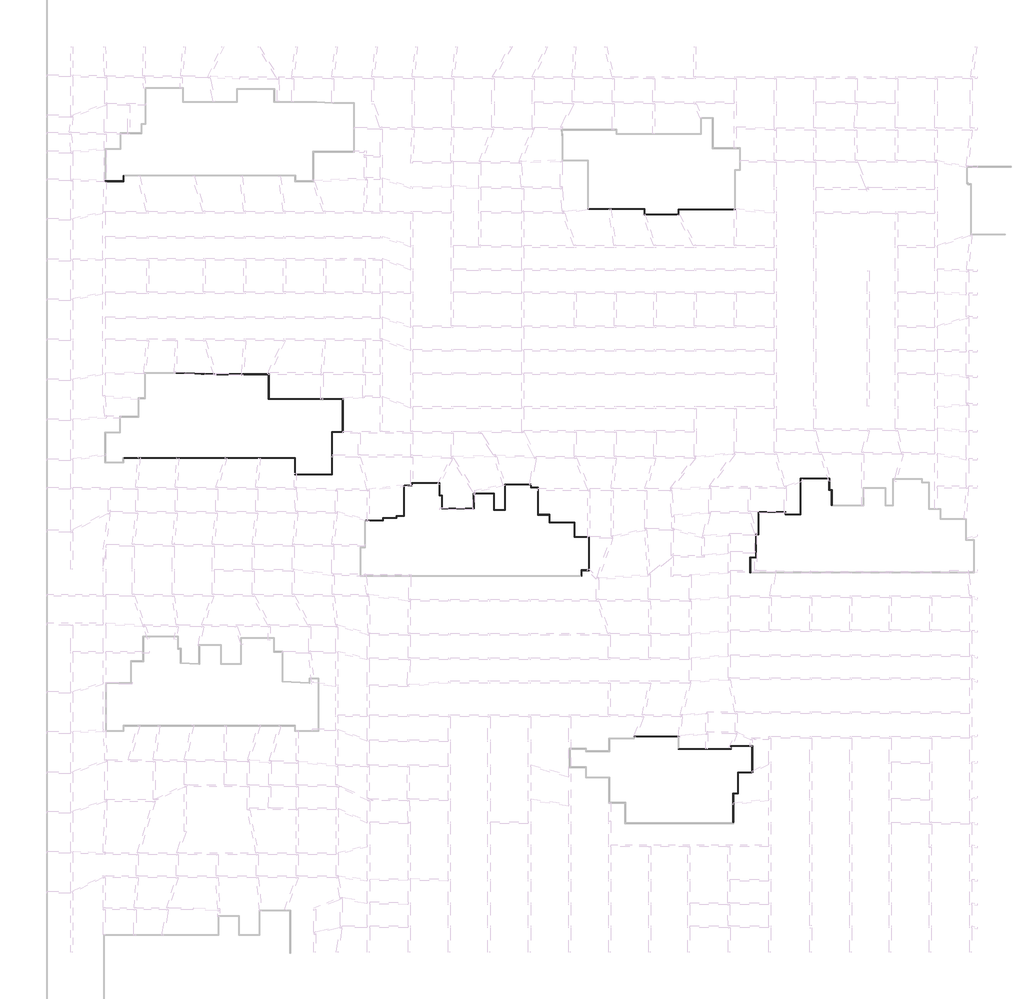
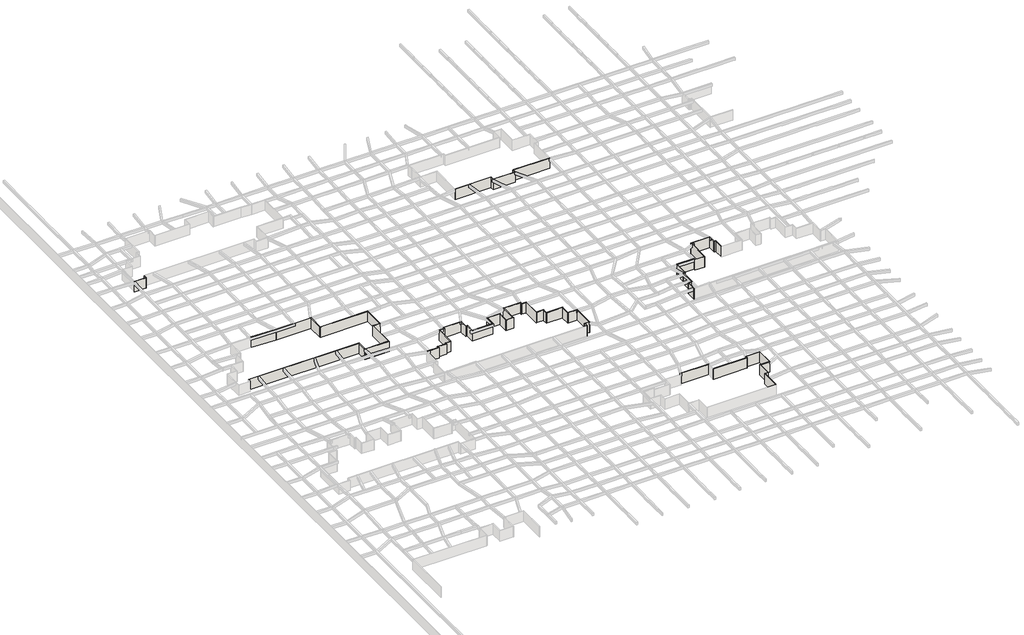
# One storey, part 6 of 45: 69 walls.
"""IFC4 building model written with IfcOpenShell, lengths in millimetres."""

from ifc_helpers import new_model, si_unit, origin, origin_with_axes, place, context, project, spatial, polyline, outline, extrude, faceted_brep, element, save

model = new_model("IFC4")

# Units and contexts
model_context = context("Model", 3, world=origin())
ifc_project = project(units=[si_unit("LENGTHUNIT", "METRE", prefix="MILLI")], contexts=[model_context])

# Site, building, storey
site = spatial("IfcSite", under=ifc_project)
building = spatial("IfcBuilding", under=site)
storey = spatial("IfcBuildingStorey", under=building, Name="户型图", Elevation=0.0)

# Walls
placement = place(None, origin())
element("IfcWall", 1, ObjectType="所有墙体", at=placement, inside=storey, context=model_context, shape_type="Brep", body=[
    faceted_brep([(-140203.5692432, 133175.8564831, 0.0), (-140203.5692432, 132195.8564831, 0.0), (-140203.5692432, 132075.8564831, 0.0), (-140203.5692432, 132075.8564831, 3300.0), (-140203.5692432, 132195.8564831, 3300.0), (-140203.5692432, 133175.8564831, 3300.0), (-140083.5692432, 133175.8564831, 0.0), (-140083.5692432, 133175.8564831, 3300.0), (-140083.5692432, 132075.8564831, 3300.0), (-140083.5692432, 132075.8564831, 0.0)], [[[0, 1, 2, 3, 4, 5]], [[6, 7, 8, 9]], [[2, 1, 0, 6, 9]], [[5, 4, 3, 8, 7]], [[0, 5, 7, 6]], [[3, 2, 9, 8]]]),
])
element("IfcWall", 2, ObjectType="所有墙体", at=placement, inside=storey, context=model_context, shape_type="Brep", body=[
    faceted_brep([(-140203.5692432, 132195.8564831, 0.0), (-143583.5692432, 132195.8564831, 0.0), (-143703.5692432, 132195.8564831, 0.0), (-143703.5692432, 132195.8564831, 3300.0), (-143583.5692432, 132195.8564831, 3300.0), (-140203.5692432, 132195.8564831, 3300.0), (-140203.5692432, 132075.8564831, 0.0), (-140203.5692432, 132075.8564831, 3300.0), (-143703.5692432, 132075.8564831, 3300.0), (-143703.5692432, 132075.8564831, 0.0)], [[[0, 1, 2, 3, 4, 5]], [[6, 7, 8, 9]], [[2, 1, 0, 6, 9]], [[5, 4, 3, 8, 7]], [[0, 5, 7, 6]], [[3, 2, 9, 8]]]),
])
element("IfcWall", 3, ObjectType="所有墙体", at=placement, inside=storey, context=model_context, shape_type="Brep", body=[
    faceted_brep([(-140131.3875586, 78294.2865852, 0.0), (-106851.3875586, 78294.2865852, 0.0), (-106731.3875586, 78294.2865852, 0.0), (-106731.3875586, 78294.2865852, 3300.0), (-106851.3875586, 78294.2865852, 3300.0), (-140131.3875586, 78294.2865852, 3300.0), (-140131.3875586, 78414.2865852, 0.0), (-140131.3875586, 78414.2865852, 3300.0), (-106731.3875586, 78414.2865852, 3300.0), (-106731.3875586, 78414.2865852, 0.0)], [[[0, 1, 2, 3, 4, 5]], [[6, 7, 8, 9]], [[2, 1, 0, 6, 9]], [[5, 4, 3, 8, 7]], [[0, 5, 7, 6]], [[3, 2, 9, 8]]]),
])
element("IfcWall", 4, ObjectType="所有墙体", at=placement, inside=storey, context=model_context, shape_type="Brep", body=[
    faceted_brep([(-106851.3875586, 78294.2865852, 0.0), (-106851.3875586, 75094.2865852, 0.0), (-106851.3875586, 75094.2865852, 3300.0), (-106851.3875586, 78294.2865852, 3300.0), (-106731.3875586, 78294.2865852, 0.0), (-106731.3875586, 78294.2865852, 3300.0), (-106731.3875586, 75214.2865852, 3300.0), (-106731.3875586, 75094.2865852, 3300.0), (-106731.3875586, 75094.2865852, 0.0), (-106731.3875586, 75214.2865852, 0.0)], [[[0, 1, 2, 3]], [[4, 5, 6, 7, 8, 9]], [[1, 0, 4, 9, 8]], [[3, 2, 7, 6, 5]], [[0, 3, 5, 4]], [[2, 1, 8, 7]]]),
])
element("IfcWall", 5, ObjectType="所有墙体", at=placement, inside=storey, context=model_context, shape_type="Brep", body=[
    faceted_brep([(-106731.3875586, 75094.2865852, 0.0), (-99531.3875586, 75094.2865852, 0.0), (-99531.3875586, 75094.2865852, 3300.0), (-106731.3875586, 75094.2865852, 3300.0), (-106731.3875586, 75214.2865852, 0.0), (-106731.3875586, 75214.2865852, 3300.0), (-99651.3875586, 75214.2865852, 3300.0), (-99531.3875586, 75214.2865852, 3300.0), (-99531.3875586, 75214.2865852, 0.0), (-99651.3875586, 75214.2865852, 0.0)], [[[0, 1, 2, 3]], [[4, 5, 6, 7, 8, 9]], [[1, 0, 4, 9, 8]], [[3, 2, 7, 6, 5]], [[0, 3, 5, 4]], [[2, 1, 8, 7]]]),
])
element("IfcWall", 6, ObjectType="所有墙体", at=placement, inside=storey, context=model_context, shape_type="Brep", body=[
    faceted_brep([(-99531.3875586, 75214.2865852, 0.0), (-99531.3875586, 83294.2865852, 0.0), (-99531.3875586, 83414.2865852, 0.0), (-99531.3875586, 83414.2865852, 3300.0), (-99531.3875586, 83294.2865852, 3300.0), (-99531.3875586, 75214.2865852, 3300.0), (-99651.3875586, 75214.2865852, 0.0), (-99651.3875586, 75214.2865852, 3300.0), (-99651.3875586, 83414.2865852, 3300.0), (-99651.3875586, 83414.2865852, 0.0)], [[[0, 1, 2, 3, 4, 5]], [[6, 7, 8, 9]], [[2, 1, 0, 6, 9]], [[5, 4, 3, 8, 7]], [[0, 5, 7, 6]], [[3, 2, 9, 8]]]),
])
element("IfcWall", 7, ObjectType="所有墙体", at=placement, inside=storey, context=model_context, shape_type="Brep", body=[
    faceted_brep([(-99531.3875586, 83294.2865852, 0.0), (-97431.3875586, 83294.2865852, 0.0), (-97431.3875586, 83294.2865852, 3300.0), (-99531.3875586, 83294.2865852, 3300.0), (-99531.3875586, 83414.2865852, 0.0), (-99531.3875586, 83414.2865852, 3300.0), (-97551.3875586, 83414.2865852, 3300.0), (-97431.3875586, 83414.2865852, 3300.0), (-97431.3875586, 83414.2865852, 0.0), (-97551.3875586, 83414.2865852, 0.0)], [[[0, 1, 2, 3]], [[4, 5, 6, 7, 8, 9]], [[1, 0, 4, 9, 8]], [[3, 2, 7, 6, 5]], [[0, 3, 5, 4]], [[2, 1, 8, 7]]]),
])
element("IfcWall", 8, ObjectType="所有墙体", at=placement, inside=storey, context=model_context, shape_type="Brep", body=[
    faceted_brep([(-97431.3875586, 83414.2865852, 0.0), (-97431.3875586, 89872.92078, 0.0), (-97431.3875586, 89872.92078, 3300.0), (-97431.3875586, 83414.2865852, 3300.0), (-97551.3875586, 83414.2865852, 0.0), (-97551.3875586, 83414.2865852, 3300.0), (-97551.3875586, 89752.92078, 3300.0), (-97551.3875586, 89872.92078, 3300.0), (-97551.3875586, 89872.92078, 0.0), (-97551.3875586, 89752.92078, 0.0)], [[[0, 1, 2, 3]], [[4, 5, 6, 7, 8, 9]], [[1, 0, 4, 9, 8]], [[3, 2, 7, 6, 5]], [[0, 3, 5, 4]], [[2, 1, 8, 7]]]),
])
element("IfcWall", 9, ObjectType="所有墙体", at=placement, inside=storey, context=model_context, shape_type="Brep", body=[
    faceted_brep([(-97551.3875586, 89872.92078, 0.0), (-111831.3875586, 89872.92078, 0.0), (-111951.3875586, 89872.92078, 0.0), (-111951.3875586, 89872.92078, 3300.0), (-111831.3875586, 89872.92078, 3300.0), (-97551.3875586, 89872.92078, 3300.0), (-97551.3875586, 89752.92078, 0.0), (-97551.3875586, 89752.92078, 3300.0), (-111951.3875586, 89752.92078, 3300.0), (-111951.3875586, 89752.92078, 0.0)], [[[0, 1, 2, 3, 4, 5]], [[6, 7, 8, 9]], [[2, 1, 0, 6, 9]], [[5, 4, 3, 8, 7]], [[0, 5, 7, 6]], [[3, 2, 9, 8]]]),
])
element("IfcWall", 10, ObjectType="所有墙体", at=placement, inside=storey, context=model_context, shape_type="Brep", body=[
    faceted_brep([(-111831.3875586, 89872.92078, 0.0), (-111831.3875586, 94672.92078, 0.0), (-111831.3875586, 94672.92078, 3300.0), (-111831.3875586, 89872.92078, 3300.0), (-111951.3875586, 89872.92078, 0.0), (-111951.3875586, 89872.92078, 3300.0), (-111951.3875586, 94552.92078, 3300.0), (-111951.3875586, 94672.92078, 3300.0), (-111951.3875586, 94672.92078, 0.0), (-111951.3875586, 94552.92078, 0.0)], [[[0, 1, 2, 3]], [[4, 5, 6, 7, 8, 9]], [[1, 0, 4, 9, 8]], [[3, 2, 7, 6, 5]], [[0, 3, 5, 4]], [[2, 1, 8, 7]]]),
])
element("IfcWall", 11, ObjectType="所有墙体", at=placement, inside=storey, context=model_context, shape_type="SweptSolid", body=[
    extrude(outline(polyline([(-122490.3402547, 94672.92078), (-111951.3875586, 94672.92078), (-111951.3875586, 94552.92078), (-122492.4348625, 94552.92078), (-122490.3402547, 94672.92078)])), origin_with_axes(), (0.0, 0.0, 1.0), 3300.0),
])
element("IfcWall", 12, ObjectType="所有墙体", at=placement, inside=storey, context=model_context, shape_type="SweptSolid", body=[
    extrude(outline(polyline([(-129985.7714573, 94934.6670053), (-122490.3402547, 94672.92078), (-122492.4348625, 94552.92078), (-129987.8660651, 94814.6670053), (-129985.7714573, 94934.6670053)])), origin_with_axes(), (0.0, 0.0, 1.0), 3300.0),
])
element("IfcWall", 13, ObjectType="所有墙体", at=placement, inside=storey, context=model_context, shape_type="Brep", body=[
    faceted_brep([(-49787.1090692, 126702.9605472, 0.0), (-38907.1090692, 126702.9605472, 0.0), (-38787.1090692, 126702.9605472, 0.0), (-38787.1090692, 126702.9605472, 3300.0), (-38907.1090692, 126702.9605472, 3300.0), (-49787.1090692, 126702.9605472, 3300.0), (-49787.1090692, 126822.9605472, 0.0), (-49787.1090692, 126822.9605472, 3300.0), (-38787.1090692, 126822.9605472, 3300.0), (-38787.1090692, 126822.9605472, 0.0)], [[[0, 1, 2, 3, 4, 5]], [[6, 7, 8, 9]], [[2, 1, 0, 6, 9]], [[5, 4, 3, 8, 7]], [[0, 5, 7, 6]], [[3, 2, 9, 8]]]),
])
element("IfcWall", 14, ObjectType="所有墙体", at=placement, inside=storey, context=model_context, shape_type="Brep", body=[
    faceted_brep([(-38907.1090692, 126702.9605472, 0.0), (-38907.1090692, 125602.9605472, 0.0), (-38907.1090692, 125602.9605472, 3300.0), (-38907.1090692, 126702.9605472, 3300.0), (-38787.1090692, 126702.9605472, 0.0), (-38787.1090692, 126702.9605472, 3300.0), (-38787.1090692, 125722.9605472, 3300.0), (-38787.1090692, 125602.9605472, 3300.0), (-38787.1090692, 125602.9605472, 0.0), (-38787.1090692, 125722.9605472, 0.0)], [[[0, 1, 2, 3]], [[4, 5, 6, 7, 8, 9]], [[1, 0, 4, 9, 8]], [[3, 2, 7, 6, 5]], [[0, 3, 5, 4]], [[2, 1, 8, 7]]]),
])
element("IfcWall", 15, ObjectType="所有墙体", at=placement, inside=storey, context=model_context, shape_type="Brep", body=[
    faceted_brep([(-38787.1090692, 125602.9605472, 0.0), (-32187.1090692, 125602.9605472, 0.0), (-32187.1090692, 125602.9605472, 3300.0), (-38787.1090692, 125602.9605472, 3300.0), (-38787.1090692, 125722.9605472, 0.0), (-38787.1090692, 125722.9605472, 3300.0), (-32307.1090692, 125722.9605472, 3300.0), (-32187.1090692, 125722.9605472, 3300.0), (-32187.1090692, 125722.9605472, 0.0), (-32307.1090692, 125722.9605472, 0.0)], [[[0, 1, 2, 3]], [[4, 5, 6, 7, 8, 9]], [[1, 0, 4, 9, 8]], [[3, 2, 7, 6, 5]], [[0, 3, 5, 4]], [[2, 1, 8, 7]]]),
])
element("IfcWall", 16, ObjectType="所有墙体", at=placement, inside=storey, context=model_context, shape_type="Brep", body=[
    faceted_brep([(-32187.1090692, 125722.9605472, 0.0), (-32187.1090692, 126602.9605472, 0.0), (-32187.1090692, 126722.9605472, 0.0), (-32187.1090692, 126722.9605472, 3300.0), (-32187.1090692, 126602.9605472, 3300.0), (-32187.1090692, 125722.9605472, 3300.0), (-32307.1090692, 125722.9605472, 0.0), (-32307.1090692, 125722.9605472, 3300.0), (-32307.1090692, 126722.9605472, 3300.0), (-32307.1090692, 126722.9605472, 0.0)], [[[0, 1, 2, 3, 4, 5]], [[6, 7, 8, 9]], [[2, 1, 0, 6, 9]], [[5, 4, 3, 8, 7]], [[0, 5, 7, 6]], [[3, 2, 9, 8]]]),
])
element("IfcWall", 17, ObjectType="所有墙体", at=placement, inside=storey, context=model_context, shape_type="Brep", body=[
    faceted_brep([(-32187.1090692, 126602.9605472, 0.0), (-21187.1090692, 126602.9605472, 0.0), (-21187.1090692, 126602.9605472, 3300.0), (-32187.1090692, 126602.9605472, 3300.0), (-32187.1090692, 126722.9605472, 0.0), (-32187.1090692, 126722.9605472, 3300.0), (-21307.1090692, 126722.9605472, 3300.0), (-21187.1090692, 126722.9605472, 3300.0), (-21187.1090692, 126722.9605472, 0.0), (-21307.1090692, 126722.9605472, 0.0)], [[[0, 1, 2, 3]], [[4, 5, 6, 7, 8, 9]], [[1, 0, 4, 9, 8]], [[3, 2, 7, 6, 5]], [[0, 3, 5, 4]], [[2, 1, 8, 7]]]),
])
element("IfcWall", 18, ObjectType="所有墙体", at=placement, inside=storey, context=model_context, shape_type="Brep", body=[
    faceted_brep([(-93093.897353, 66089.1206587, 0.0), (-89610.9508463, 66089.1206587, 0.0), (-89610.9508463, 66089.1206587, 3300.0), (-93093.897353, 66089.1206587, 3300.0), (-93093.897353, 66209.1206587, 0.0), (-93093.897353, 66209.1206587, 3300.0), (-89730.9508463, 66209.1206587, 3300.0), (-89610.9508463, 66209.1206587, 3300.0), (-89610.9508463, 66209.1206587, 0.0), (-89730.9508463, 66209.1206587, 0.0)], [[[0, 1, 2, 3]], [[4, 5, 6, 7, 8, 9]], [[1, 0, 4, 9, 8]], [[3, 2, 7, 6, 5]], [[2, 1, 8, 7]], [[0, 3, 5, 4]]]),
])
element("IfcWall", 19, ObjectType="所有墙体", at=placement, inside=storey, context=model_context, shape_type="Brep", body=[
    faceted_brep([(-89610.9508463, 66209.1206587, 0.0), (-89610.9508463, 66589.1206587, 0.0), (-89610.9508463, 66709.1206587, 0.0), (-89610.9508463, 66709.1206587, 3300.0), (-89610.9508463, 66589.1206587, 3300.0), (-89610.9508463, 66209.1206587, 3300.0), (-89730.9508463, 66209.1206587, 0.0), (-89730.9508463, 66209.1206587, 3300.0), (-89730.9508463, 66709.1206587, 3300.0), (-89730.9508463, 66709.1206587, 0.0)], [[[0, 1, 2, 3, 4, 5]], [[6, 7, 8, 9]], [[2, 1, 0, 6, 9]], [[5, 4, 3, 8, 7]], [[0, 5, 7, 6]], [[3, 2, 9, 8]]]),
])
element("IfcWall", 20, ObjectType="所有墙体", at=placement, inside=storey, context=model_context, shape_type="Brep", body=[
    faceted_brep([(-89610.9508463, 66589.1206587, 0.0), (-87010.9508463, 66589.1206587, 0.0), (-87010.9508463, 66589.1206587, 3300.0), (-89610.9508463, 66589.1206587, 3300.0), (-89610.9508463, 66709.1206587, 0.0), (-89610.9508463, 66709.1206587, 3300.0), (-87130.9508463, 66709.1206587, 3300.0), (-87010.9508463, 66709.1206587, 3300.0), (-87010.9508463, 66709.1206587, 0.0), (-87130.9508463, 66709.1206587, 0.0)], [[[0, 1, 2, 3]], [[4, 5, 6, 7, 8, 9]], [[1, 0, 4, 9, 8]], [[3, 2, 7, 6, 5]], [[0, 3, 5, 4]], [[2, 1, 8, 7]]]),
])
element("IfcWall", 21, ObjectType="所有墙体", at=placement, inside=storey, context=model_context, shape_type="Brep", body=[
    faceted_brep([(-87010.9508463, 66709.1206587, 0.0), (-87010.9508463, 66989.1206587, 0.0), (-87010.9508463, 67109.1206587, 0.0), (-87010.9508463, 67109.1206587, 3300.0), (-87010.9508463, 66989.1206587, 3300.0), (-87010.9508463, 66709.1206587, 3300.0), (-87130.9508463, 66709.1206587, 0.0), (-87130.9508463, 66709.1206587, 3300.0), (-87130.9508463, 67109.1206587, 3300.0), (-87130.9508463, 67109.1206587, 0.0)], [[[0, 1, 2, 3, 4, 5]], [[6, 7, 8, 9]], [[2, 1, 0, 6, 9]], [[5, 4, 3, 8, 7]], [[0, 5, 7, 6]], [[3, 2, 9, 8]]]),
])
element("IfcWall", 22, ObjectType="所有墙体", at=placement, inside=storey, context=model_context, shape_type="Brep", body=[
    faceted_brep([(-87010.9508463, 66989.1206587, 0.0), (-85510.9508463, 66989.1206587, 0.0), (-85510.9508463, 66989.1206587, 3300.0), (-87010.9508463, 66989.1206587, 3300.0), (-87010.9508463, 67109.1206587, 0.0), (-87010.9508463, 67109.1206587, 3300.0), (-85630.9508463, 67109.1206587, 3300.0), (-85510.9508463, 67109.1206587, 3300.0), (-85510.9508463, 67109.1206587, 0.0), (-85630.9508463, 67109.1206587, 0.0)], [[[0, 1, 2, 3]], [[4, 5, 6, 7, 8, 9]], [[1, 0, 4, 9, 8]], [[3, 2, 7, 6, 5]], [[0, 3, 5, 4]], [[2, 1, 8, 7]]]),
])
element("IfcWall", 23, ObjectType="所有墙体", at=placement, inside=storey, context=model_context, shape_type="Brep", body=[
    faceted_brep([(-85510.9508463, 67109.1206587, 0.0), (-85510.9508463, 72887.1913736, 0.0), (-85510.9508463, 73007.1913736, 0.0), (-85510.9508463, 73007.1913736, 3300.0), (-85510.9508463, 72887.1913736, 3300.0), (-85510.9508463, 67109.1206587, 3300.0), (-85630.9508463, 67109.1206587, 0.0), (-85630.9508463, 67109.1206587, 3300.0), (-85630.9508463, 73007.1913736, 3300.0), (-85630.9508463, 73007.1913736, 0.0)], [[[0, 1, 2, 3, 4, 5]], [[6, 7, 8, 9]], [[2, 1, 0, 6, 9]], [[5, 4, 3, 8, 7]], [[0, 5, 7, 6]], [[3, 2, 9, 8]]]),
])
element("IfcWall", 24, ObjectType="所有墙体", at=placement, inside=storey, context=model_context, shape_type="Brep", body=[
    faceted_brep([(-85510.9508463, 72887.1913736, 0.0), (-84010.9508463, 72887.1913736, 0.0), (-84010.9508463, 72887.1913736, 3300.0), (-85510.9508463, 72887.1913736, 3300.0), (-85510.9508463, 73007.1913736, 0.0), (-85510.9508463, 73007.1913736, 3300.0), (-84130.9508463, 73007.1913736, 3300.0), (-84010.9508463, 73007.1913736, 3300.0), (-84010.9508463, 73007.1913736, 0.0), (-84130.9508463, 73007.1913736, 0.0)], [[[0, 1, 2, 3]], [[4, 5, 6, 7, 8, 9]], [[1, 0, 4, 9, 8]], [[3, 2, 7, 6, 5]], [[0, 3, 5, 4]], [[2, 1, 8, 7]]]),
])
element("IfcWall", 25, ObjectType="所有墙体", at=placement, inside=storey, context=model_context, shape_type="Brep", body=[
    faceted_brep([(-84010.9508463, 73007.1913736, 0.0), (-84010.9508463, 73387.1913736, 0.0), (-84010.9508463, 73507.1913736, 0.0), (-84010.9508463, 73507.1913736, 3300.0), (-84010.9508463, 73387.1913736, 3300.0), (-84010.9508463, 73007.1913736, 3300.0), (-84130.9508463, 73007.1913736, 0.0), (-84130.9508463, 73007.1913736, 3300.0), (-84130.9508463, 73507.1913736, 3300.0), (-84130.9508463, 73507.1913736, 0.0)], [[[0, 1, 2, 3, 4, 5]], [[6, 7, 8, 9]], [[2, 1, 0, 6, 9]], [[5, 4, 3, 8, 7]], [[0, 5, 7, 6]], [[3, 2, 9, 8]]]),
])
element("IfcWall", 26, ObjectType="所有墙体", at=placement, inside=storey, context=model_context, shape_type="Brep", body=[
    faceted_brep([(-84010.9508463, 73387.1913736, 0.0), (-78767.8659344, 73387.1913736, 0.0), (-78647.8659344, 73387.1913736, 0.0), (-78647.8659344, 73387.1913736, 3300.0), (-78767.8659344, 73387.1913736, 3300.0), (-84010.9508463, 73387.1913736, 3300.0), (-84010.9508463, 73507.1913736, 0.0), (-84010.9508463, 73507.1913736, 3300.0), (-78647.8659344, 73507.1913736, 3300.0), (-78647.8659344, 73507.1913736, 0.0)], [[[0, 1, 2, 3, 4, 5]], [[6, 7, 8, 9]], [[2, 1, 0, 6, 9]], [[5, 4, 3, 8, 7]], [[0, 5, 7, 6]], [[3, 2, 9, 8]]]),
])
element("IfcWall", 27, ObjectType="所有墙体", at=placement, inside=storey, context=model_context, shape_type="Brep", body=[
    faceted_brep([(-78767.8659344, 73387.1913736, 0.0), (-78767.8659344, 70987.1913736, 0.0), (-78767.8659344, 70987.1913736, 3300.0), (-78767.8659344, 73387.1913736, 3300.0), (-78647.8659344, 73387.1913736, 0.0), (-78647.8659344, 73387.1913736, 3300.0), (-78647.8659344, 71107.1913736, 3300.0), (-78647.8659344, 70987.1913736, 3300.0), (-78647.8659344, 70987.1913736, 0.0), (-78647.8659344, 71107.1913736, 0.0)], [[[0, 1, 2, 3]], [[4, 5, 6, 7, 8, 9]], [[1, 0, 4, 9, 8]], [[3, 2, 7, 6, 5]], [[0, 3, 5, 4]], [[2, 1, 8, 7]]]),
])
element("IfcWall", 28, ObjectType="所有墙体", at=placement, inside=storey, context=model_context, shape_type="Brep", body=[
    faceted_brep([(-78647.8659344, 70987.1913736, 0.0), (-78267.8659344, 70987.1913736, 0.0), (-78147.8659344, 70987.1913736, 0.0), (-78147.8659344, 70987.1913736, 3300.0), (-78267.8659344, 70987.1913736, 3300.0), (-78647.8659344, 70987.1913736, 3300.0), (-78647.8659344, 71107.1913736, 0.0), (-78647.8659344, 71107.1913736, 3300.0), (-78147.8659344, 71107.1913736, 3300.0), (-78147.8659344, 71107.1913736, 0.0)], [[[0, 1, 2, 3, 4, 5]], [[6, 7, 8, 9]], [[2, 1, 0, 6, 9]], [[5, 4, 3, 8, 7]], [[0, 5, 7, 6]], [[3, 2, 9, 8]]]),
])
element("IfcWall", 29, ObjectType="所有墙体", at=placement, inside=storey, context=model_context, shape_type="Brep", body=[
    faceted_brep([(-78267.8659344, 70987.1913736, 0.0), (-78267.8659344, 68427.6131193, 0.0), (-78267.8659344, 68427.6131193, 3300.0), (-78267.8659344, 70987.1913736, 3300.0), (-78147.8659344, 70987.1913736, 0.0), (-78147.8659344, 70987.1913736, 3300.0), (-78147.8659344, 68547.6131193, 3300.0), (-78147.8659344, 68427.6131193, 3300.0), (-78147.8659344, 68427.6131193, 0.0), (-78147.8659344, 68547.6131193, 0.0)], [[[0, 1, 2, 3]], [[4, 5, 6, 7, 8, 9]], [[1, 0, 4, 9, 8]], [[3, 2, 7, 6, 5]], [[0, 3, 5, 4]], [[2, 1, 8, 7]]]),
])
element("IfcWall", 30, ObjectType="所有墙体", at=placement, inside=storey, context=model_context, shape_type="Brep", body=[
    faceted_brep([(-78147.8659344, 68427.6131193, 0.0), (-71958.8192159, 68427.6131193, 0.0), (-71958.8192159, 68427.6131193, 3300.0), (-78147.8659344, 68427.6131193, 3300.0), (-78147.8659344, 68547.6131193, 0.0), (-78147.8659344, 68547.6131193, 3300.0), (-72078.8192159, 68547.6131193, 3300.0), (-71958.8192159, 68547.6131193, 3300.0), (-71958.8192159, 68547.6131193, 0.0), (-72078.8192159, 68547.6131193, 0.0)], [[[0, 1, 2, 3]], [[4, 5, 6, 7, 8, 9]], [[1, 0, 4, 9, 8]], [[3, 2, 7, 6, 5]], [[0, 3, 5, 4]], [[2, 1, 8, 7]]]),
])
element("IfcWall", 31, ObjectType="所有墙体", at=placement, inside=storey, context=model_context, shape_type="Brep", body=[
    faceted_brep([(-71958.8192159, 68547.6131193, 0.0), (-71958.8192159, 71355.8858644, 0.0), (-71958.8192159, 71475.8858644, 0.0), (-71958.8192159, 71475.8858644, 3300.0), (-71958.8192159, 71355.8858644, 3300.0), (-71958.8192159, 68547.6131193, 3300.0), (-72078.8192159, 68547.6131193, 0.0), (-72078.8192159, 68547.6131193, 3300.0), (-72078.8192159, 71475.8858644, 3300.0), (-72078.8192159, 71475.8858644, 0.0)], [[[0, 1, 2, 3, 4, 5]], [[6, 7, 8, 9]], [[2, 1, 0, 6, 9]], [[5, 4, 3, 8, 7]], [[0, 5, 7, 6]], [[3, 2, 9, 8]]]),
])
element("IfcWall", 32, ObjectType="所有墙体", at=placement, inside=storey, context=model_context, shape_type="Brep", body=[
    faceted_brep([(-71958.8192159, 71355.8858644, 0.0), (-68178.8192159, 71355.8858644, 0.0), (-68058.8192159, 71355.8858644, 0.0), (-68058.8192159, 71355.8858644, 3300.0), (-68178.8192159, 71355.8858644, 3300.0), (-71958.8192159, 71355.8858644, 3300.0), (-71958.8192159, 71475.8858644, 0.0), (-71958.8192159, 71475.8858644, 3300.0), (-68058.8192159, 71475.8858644, 3300.0), (-68058.8192159, 71475.8858644, 0.0)], [[[0, 1, 2, 3, 4, 5]], [[6, 7, 8, 9]], [[2, 1, 0, 6, 9]], [[5, 4, 3, 8, 7]], [[0, 5, 7, 6]], [[3, 2, 9, 8]]]),
])
element("IfcWall", 33, ObjectType="所有墙体", at=placement, inside=storey, context=model_context, shape_type="Brep", body=[
    faceted_brep([(-68178.8192159, 71355.8858644, 0.0), (-68178.8192159, 68155.8858644, 0.0), (-68178.8192159, 68155.8858644, 3300.0), (-68178.8192159, 71355.8858644, 3300.0), (-68058.8192159, 71355.8858644, 0.0), (-68058.8192159, 71355.8858644, 3300.0), (-68058.8192159, 68275.8858644, 3300.0), (-68058.8192159, 68155.8858644, 3300.0), (-68058.8192159, 68155.8858644, 0.0), (-68058.8192159, 68275.8858644, 0.0)], [[[0, 1, 2, 3]], [[4, 5, 6, 7, 8, 9]], [[1, 0, 4, 9, 8]], [[3, 2, 7, 6, 5]], [[0, 3, 5, 4]], [[2, 1, 8, 7]]]),
])
element("IfcWall", 34, ObjectType="所有墙体", at=placement, inside=storey, context=model_context, shape_type="Brep", body=[
    faceted_brep([(-68058.8192159, 68155.8858644, 0.0), (-65858.8192159, 68155.8858644, 0.0), (-65858.8192159, 68155.8858644, 3300.0), (-68058.8192159, 68155.8858644, 3300.0), (-68058.8192159, 68275.8858644, 0.0), (-68058.8192159, 68275.8858644, 3300.0), (-65978.8192159, 68275.8858644, 3300.0), (-65858.8192159, 68275.8858644, 3300.0), (-65858.8192159, 68275.8858644, 0.0), (-65978.8192159, 68275.8858644, 0.0)], [[[0, 1, 2, 3]], [[4, 5, 6, 7, 8, 9]], [[1, 0, 4, 9, 8]], [[3, 2, 7, 6, 5]], [[0, 3, 5, 4]], [[2, 1, 8, 7]]]),
])
element("IfcWall", 35, ObjectType="所有墙体", at=placement, inside=storey, context=model_context, shape_type="Brep", body=[
    faceted_brep([(-65858.8192159, 68275.8858644, 0.0), (-65858.8192159, 73135.9090851, 0.0), (-65858.8192159, 73255.9090851, 0.0), (-65858.8192159, 73255.9090851, 3300.0), (-65858.8192159, 73135.9090851, 3300.0), (-65858.8192159, 68275.8858644, 3300.0), (-65978.8192159, 68275.8858644, 0.0), (-65978.8192159, 68275.8858644, 3300.0), (-65978.8192159, 73255.9090851, 3300.0), (-65978.8192159, 73255.9090851, 0.0)], [[[0, 1, 2, 3, 4, 5]], [[6, 7, 8, 9]], [[2, 1, 0, 6, 9]], [[5, 4, 3, 8, 7]], [[0, 5, 7, 6]], [[3, 2, 9, 8]]]),
])
element("IfcWall", 36, ObjectType="所有墙体", at=placement, inside=storey, context=model_context, shape_type="Brep", body=[
    faceted_brep([(-65858.8192159, 73135.9090851, 0.0), (-60973.897353, 73135.9090851, 0.0), (-60853.897353, 73135.9090851, 0.0), (-60853.897353, 73135.9090851, 3300.0), (-60973.897353, 73135.9090851, 3300.0), (-65858.8192159, 73135.9090851, 3300.0), (-65858.8192159, 73255.9090851, 0.0), (-65858.8192159, 73255.9090851, 3300.0), (-60853.897353, 73255.9090851, 3300.0), (-60853.897353, 73255.9090851, 0.0)], [[[0, 1, 2, 3, 4, 5]], [[6, 7, 8, 9]], [[2, 1, 0, 6, 9]], [[5, 4, 3, 8, 7]], [[0, 5, 7, 6]], [[3, 2, 9, 8]]]),
])
element("IfcWall", 37, ObjectType="所有墙体", at=placement, inside=storey, context=model_context, shape_type="Brep", body=[
    faceted_brep([(-60973.897353, 73135.9090851, 0.0), (-60973.897353, 72535.9090851, 0.0), (-60973.897353, 72535.9090851, 3300.0), (-60973.897353, 73135.9090851, 3300.0), (-60853.897353, 73135.9090851, 0.0), (-60853.897353, 73135.9090851, 3300.0), (-60853.897353, 72655.9090851, 3300.0), (-60853.897353, 72535.9090851, 3300.0), (-60853.897353, 72535.9090851, 0.0), (-60853.897353, 72655.9090851, 0.0)], [[[0, 1, 2, 3]], [[4, 5, 6, 7, 8, 9]], [[1, 0, 4, 9, 8]], [[3, 2, 7, 6, 5]], [[0, 3, 5, 4]], [[2, 1, 8, 7]]]),
])
element("IfcWall", 38, ObjectType="所有墙体", at=placement, inside=storey, context=model_context, shape_type="Brep", body=[
    faceted_brep([(-60853.897353, 72535.9090851, 0.0), (-59573.897353, 72535.9090851, 0.0), (-59453.897353, 72535.9090851, 0.0), (-59453.897353, 72535.9090851, 3300.0), (-59573.897353, 72535.9090851, 3300.0), (-60853.897353, 72535.9090851, 3300.0), (-60853.897353, 72655.9090851, 0.0), (-60853.897353, 72655.9090851, 3300.0), (-59453.897353, 72655.9090851, 3300.0), (-59453.897353, 72655.9090851, 0.0)], [[[0, 1, 2, 3, 4, 5]], [[6, 7, 8, 9]], [[2, 1, 0, 6, 9]], [[5, 4, 3, 8, 7]], [[0, 5, 7, 6]], [[3, 2, 9, 8]]]),
])
element("IfcWall", 39, ObjectType="所有墙体", at=placement, inside=storey, context=model_context, shape_type="Brep", body=[
    faceted_brep([(-59573.897353, 72535.9090851, 0.0), (-59573.897353, 67235.9090851, 0.0), (-59573.897353, 67235.9090851, 3300.0), (-59573.897353, 72535.9090851, 3300.0), (-59453.897353, 72535.9090851, 0.0), (-59453.897353, 72535.9090851, 3300.0), (-59453.897353, 67355.9090851, 3300.0), (-59453.897353, 67235.9090851, 3300.0), (-59453.897353, 67235.9090851, 0.0), (-59453.897353, 67355.9090851, 0.0)], [[[0, 1, 2, 3]], [[4, 5, 6, 7, 8, 9]], [[1, 0, 4, 9, 8]], [[3, 2, 7, 6, 5]], [[0, 3, 5, 4]], [[2, 1, 8, 7]]]),
])
element("IfcWall", 40, ObjectType="所有墙体", at=placement, inside=storey, context=model_context, shape_type="Brep", body=[
    faceted_brep([(-59453.897353, 67235.9090851, 0.0), (-57373.897353, 67235.9090851, 0.0), (-57253.897353, 67235.9090851, 0.0), (-57253.897353, 67235.9090851, 3300.0), (-57373.897353, 67235.9090851, 3300.0), (-59453.897353, 67235.9090851, 3300.0), (-59453.897353, 67355.9090851, 0.0), (-59453.897353, 67355.9090851, 3300.0), (-57253.897353, 67355.9090851, 3300.0), (-57253.897353, 67355.9090851, 0.0)], [[[0, 1, 2, 3, 4, 5]], [[6, 7, 8, 9]], [[2, 1, 0, 6, 9]], [[5, 4, 3, 8, 7]], [[0, 5, 7, 6]], [[3, 2, 9, 8]]]),
])
element("IfcWall", 41, ObjectType="所有墙体", at=placement, inside=storey, context=model_context, shape_type="Brep", body=[
    faceted_brep([(-57373.897353, 67235.9090851, 0.0), (-57373.897353, 65735.9090851, 0.0), (-57373.897353, 65735.9090851, 3300.0), (-57373.897353, 67235.9090851, 3300.0), (-57253.897353, 67235.9090851, 0.0), (-57253.897353, 67235.9090851, 3300.0), (-57253.897353, 65855.9090851, 3300.0), (-57253.897353, 65735.9090851, 3300.0), (-57253.897353, 65735.9090851, 0.0), (-57253.897353, 65855.9090851, 0.0)], [[[0, 1, 2, 3]], [[4, 5, 6, 7, 8, 9]], [[1, 0, 4, 9, 8]], [[3, 2, 7, 6, 5]], [[0, 3, 5, 4]], [[2, 1, 8, 7]]]),
])
element("IfcWall", 42, ObjectType="所有墙体", at=placement, inside=storey, context=model_context, shape_type="Brep", body=[
    faceted_brep([(-57253.897353, 65735.9090851, 0.0), (-52473.897353, 65735.9090851, 0.0), (-52353.897353, 65735.9090851, 0.0), (-52353.897353, 65735.9090851, 3300.0), (-52473.897353, 65735.9090851, 3300.0), (-57253.897353, 65735.9090851, 3300.0), (-57253.897353, 65855.9090851, 0.0), (-57253.897353, 65855.9090851, 3300.0), (-52353.897353, 65855.9090851, 3300.0), (-52353.897353, 65855.9090851, 0.0)], [[[0, 1, 2, 3, 4, 5]], [[6, 7, 8, 9]], [[2, 1, 0, 6, 9]], [[5, 4, 3, 8, 7]], [[0, 5, 7, 6]], [[3, 2, 9, 8]]]),
])
element("IfcWall", 43, ObjectType="所有墙体", at=placement, inside=storey, context=model_context, shape_type="Brep", body=[
    faceted_brep([(-52473.897353, 65735.9090851, 0.0), (-52473.897353, 62935.9090851, 0.0), (-52473.897353, 62935.9090851, 3300.0), (-52473.897353, 65735.9090851, 3300.0), (-52353.897353, 65735.9090851, 0.0), (-52353.897353, 65735.9090851, 3300.0), (-52353.897353, 63055.9090851, 3300.0), (-52353.897353, 62935.9090851, 3300.0), (-52353.897353, 62935.9090851, 0.0), (-52353.897353, 63055.9090851, 0.0)], [[[0, 1, 2, 3]], [[4, 5, 6, 7, 8, 9]], [[1, 0, 4, 9, 8]], [[3, 2, 7, 6, 5]], [[0, 3, 5, 4]], [[2, 1, 8, 7]]]),
])
element("IfcWall", 44, ObjectType="所有墙体", at=placement, inside=storey, context=model_context, shape_type="Brep", body=[
    faceted_brep([(-52353.897353, 62935.9090851, 0.0), (-49673.897353, 62935.9090851, 0.0), (-49553.897353, 62935.9090851, 0.0), (-49553.897353, 62935.9090851, 3300.0), (-49673.897353, 62935.9090851, 3300.0), (-52353.897353, 62935.9090851, 3300.0), (-52353.897353, 63055.9090851, 0.0), (-52353.897353, 63055.9090851, 3300.0), (-49553.897353, 63055.9090851, 3300.0), (-49553.897353, 63055.9090851, 0.0)], [[[0, 1, 2, 3, 4, 5]], [[6, 7, 8, 9]], [[2, 1, 0, 6, 9]], [[5, 4, 3, 8, 7]], [[0, 5, 7, 6]], [[3, 2, 9, 8]]]),
])
element("IfcWall", 45, ObjectType="所有墙体", at=placement, inside=storey, context=model_context, shape_type="Brep", body=[
    faceted_brep([(-49673.897353, 62935.9090851, 0.0), (-49673.897353, 56555.9851813, 0.0), (-49673.897353, 56435.9851813, 0.0), (-49673.897353, 56435.9851813, 3300.0), (-49673.897353, 56555.9851813, 3300.0), (-49673.897353, 62935.9090851, 3300.0), (-49553.897353, 62935.9090851, 0.0), (-49553.897353, 62935.9090851, 3300.0), (-49553.897353, 56435.9851813, 3300.0), (-49553.897353, 56435.9851813, 0.0)], [[[0, 1, 2, 3, 4, 5]], [[6, 7, 8, 9]], [[2, 1, 0, 6, 9]], [[5, 4, 3, 8, 7]], [[0, 5, 7, 6]], [[3, 2, 9, 8]]]),
])
element("IfcWall", 46, ObjectType="所有墙体", at=placement, inside=storey, context=model_context, shape_type="Brep", body=[
    faceted_brep([(-51113.897353, 56435.9851813, 0.0), (-50993.897353, 56435.9851813, 0.0), (-49673.897353, 56435.9851813, 0.0), (-49673.897353, 56435.9851813, 3300.0), (-50993.897353, 56435.9851813, 3300.0), (-51113.897353, 56435.9851813, 3300.0), (-51113.897353, 56555.9851813, 0.0), (-51113.897353, 56555.9851813, 3300.0), (-49673.897353, 56555.9851813, 3300.0), (-49673.897353, 56555.9851813, 0.0)], [[[0, 1, 2, 3, 4, 5]], [[6, 7, 8, 9]], [[2, 1, 0, 6, 9]], [[5, 4, 3, 8, 7]], [[3, 2, 9, 8]], [[0, 5, 7, 6]]]),
])
element("IfcWall", 47, ObjectType="所有墙体", at=placement, inside=storey, context=model_context, shape_type="Brep", body=[
    faceted_brep([(-51113.897353, 56435.9851813, 0.0), (-51113.897353, 55455.9851813, 0.0), (-51113.897353, 55335.9851813, 0.0), (-51113.897353, 55335.9851813, 3300.0), (-51113.897353, 55455.9851813, 3300.0), (-51113.897353, 56435.9851813, 3300.0), (-50993.897353, 56435.9851813, 0.0), (-50993.897353, 56435.9851813, 3300.0), (-50993.897353, 55335.9851813, 3300.0), (-50993.897353, 55335.9851813, 0.0)], [[[0, 1, 2, 3, 4, 5]], [[6, 7, 8, 9]], [[2, 1, 0, 6, 9]], [[5, 4, 3, 8, 7]], [[0, 5, 7, 6]], [[3, 2, 9, 8]]]),
])
element("IfcWall", 48, ObjectType="所有墙体", at=placement, inside=storey, context=model_context, shape_type="Brep", body=[
    faceted_brep([(-16720.9650169, 67905.9852797, 0.0), (-16720.9650169, 63565.9852797, 0.0), (-16720.9650169, 63445.9852797, 0.0), (-16720.9650169, 63445.9852797, 3300.0), (-16720.9650169, 63565.9852797, 3300.0), (-16720.9650169, 67905.9852797, 3300.0), (-16600.9650169, 67905.9852797, 0.0), (-16600.9650169, 67905.9852797, 3300.0), (-16600.9650169, 67785.9852797, 3300.0), (-16600.9650169, 63445.9852797, 3300.0), (-16600.9650169, 63445.9852797, 0.0), (-16600.9650169, 67785.9852797, 0.0)], [[[0, 1, 2, 3, 4, 5]], [[6, 7, 8, 9, 10, 11]], [[2, 1, 0, 6, 11, 10]], [[5, 4, 3, 9, 8, 7]], [[3, 2, 10, 9]], [[0, 5, 7, 6]]]),
])
element("IfcWall", 49, ObjectType="所有墙体", at=placement, inside=storey, context=model_context, shape_type="Brep", body=[
    faceted_brep([(-16720.9650169, 63565.9852797, 0.0), (-17232.8482451, 63565.9852797, 0.0), (-17232.8482451, 63565.9852797, 3300.0), (-16720.9650169, 63565.9852797, 3300.0), (-16720.9650169, 63445.9852797, 0.0), (-16720.9650169, 63445.9852797, 3300.0), (-17112.8482451, 63445.9852797, 3300.0), (-17232.8482451, 63445.9852797, 3300.0), (-17232.8482451, 63445.9852797, 0.0), (-17112.8482451, 63445.9852797, 0.0)], [[[0, 1, 2, 3]], [[4, 5, 6, 7, 8, 9]], [[1, 0, 4, 9, 8]], [[3, 2, 7, 6, 5]], [[0, 3, 5, 4]], [[2, 1, 8, 7]]]),
])
element("IfcWall", 50, ObjectType="所有墙体", at=placement, inside=storey, context=model_context, shape_type="Brep", body=[
    faceted_brep([(-17232.8482451, 63445.9852797, 0.0), (-17232.8482451, 59065.9852797, 0.0), (-17232.8482451, 58945.9852797, 0.0), (-17232.8482451, 58945.9852797, 3300.0), (-17232.8482451, 59065.9852797, 3300.0), (-17232.8482451, 63445.9852797, 3300.0), (-17112.8482451, 63445.9852797, 0.0), (-17112.8482451, 63445.9852797, 3300.0), (-17112.8482451, 58945.9852797, 3300.0), (-17112.8482451, 58945.9852797, 0.0)], [[[0, 1, 2, 3, 4, 5]], [[6, 7, 8, 9]], [[2, 1, 0, 6, 9]], [[5, 4, 3, 8, 7]], [[0, 5, 7, 6]], [[3, 2, 9, 8]]]),
])
element("IfcWall", 51, ObjectType="所有墙体", at=placement, inside=storey, context=model_context, shape_type="Brep", body=[
    faceted_brep([(-17232.8482451, 59065.9852797, 0.0), (-18332.8482451, 59065.9852797, 0.0), (-18332.8482451, 59065.9852797, 3300.0), (-17232.8482451, 59065.9852797, 3300.0), (-17232.8482451, 58945.9852797, 0.0), (-17232.8482451, 58945.9852797, 3300.0), (-18212.8482451, 58945.9852797, 3300.0), (-18332.8482451, 58945.9852797, 3300.0), (-18332.8482451, 58945.9852797, 0.0), (-18212.8482451, 58945.9852797, 0.0)], [[[0, 1, 2, 3]], [[4, 5, 6, 7, 8, 9]], [[1, 0, 4, 9, 8]], [[3, 2, 7, 6, 5]], [[0, 3, 5, 4]], [[2, 1, 8, 7]]]),
])
element("IfcWall", 52, ObjectType="所有墙体", at=placement, inside=storey, context=model_context, shape_type="Brep", body=[
    faceted_brep([(-18332.8482451, 58945.9852797, 0.0), (-18332.8482451, 56016.5180379, 0.0), (-18332.8482451, 56016.5180379, 3300.0), (-18332.8482451, 58945.9852797, 3300.0), (-18212.8482451, 58945.9852797, 0.0), (-18212.8482451, 58945.9852797, 3300.0), (-18212.8482451, 56136.5180379, 3300.0), (-18212.8482451, 56016.5180379, 3300.0), (-18212.8482451, 56016.5180379, 0.0), (-18212.8482451, 56136.5180379, 0.0)], [[[0, 1, 2, 3]], [[4, 5, 6, 7, 8, 9]], [[1, 0, 4, 9, 8]], [[3, 2, 7, 6, 5]], [[0, 3, 5, 4]], [[2, 1, 8, 7]]]),
])
element("IfcWall", 53, ObjectType="所有墙体", at=placement, inside=storey, context=model_context, shape_type="Brep", body=[
    faceted_brep([(-2351.9998188, 69132.5341829, 0.0), (-2351.9998188, 72132.5341829, 0.0), (-2351.9998188, 72132.5341829, 3300.0), (-2351.9998188, 69132.5341829, 3300.0), (-2471.9998188, 69132.5341829, 0.0), (-2471.9998188, 69132.5341829, 3300.0), (-2471.9998188, 72012.5341829, 3300.0), (-2471.9998188, 72132.5341829, 3300.0), (-2471.9998188, 72132.5341829, 0.0), (-2471.9998188, 72012.5341829, 0.0)], [[[0, 1, 2, 3]], [[4, 5, 6, 7, 8, 9]], [[1, 0, 4, 9, 8]], [[3, 2, 7, 6, 5]], [[0, 3, 5, 4]], [[2, 1, 8, 7]]]),
])
element("IfcWall", 54, ObjectType="所有墙体", at=placement, inside=storey, context=model_context, shape_type="Brep", body=[
    faceted_brep([(-2471.9998188, 72132.5341829, 0.0), (-2851.9998188, 72132.5341829, 0.0), (-2971.9998188, 72132.5341829, 0.0), (-2971.9998188, 72132.5341829, 3300.0), (-2851.9998188, 72132.5341829, 3300.0), (-2471.9998188, 72132.5341829, 3300.0), (-2471.9998188, 72012.5341829, 0.0), (-2471.9998188, 72012.5341829, 3300.0), (-2971.9998188, 72012.5341829, 3300.0), (-2971.9998188, 72012.5341829, 0.0)], [[[0, 1, 2, 3, 4, 5]], [[6, 7, 8, 9]], [[2, 1, 0, 6, 9]], [[5, 4, 3, 8, 7]], [[0, 5, 7, 6]], [[3, 2, 9, 8]]]),
])
element("IfcWall", 55, ObjectType="所有墙体", at=placement, inside=storey, context=model_context, shape_type="Brep", body=[
    faceted_brep([(-2851.9998188, 72132.5341829, 0.0), (-2851.9998188, 74437.7257306, 0.0), (-2851.9998188, 74437.7257306, 3300.0), (-2851.9998188, 72132.5341829, 3300.0), (-2971.9998188, 72132.5341829, 0.0), (-2971.9998188, 72132.5341829, 3300.0), (-2971.9998188, 74317.7257306, 3300.0), (-2971.9998188, 74437.7257306, 3300.0), (-2971.9998188, 74437.7257306, 0.0), (-2971.9998188, 74317.7257306, 0.0)], [[[0, 1, 2, 3]], [[4, 5, 6, 7, 8, 9]], [[1, 0, 4, 9, 8]], [[3, 2, 7, 6, 5]], [[0, 3, 5, 4]], [[2, 1, 8, 7]]]),
])
element("IfcWall", 56, ObjectType="所有墙体", at=placement, inside=storey, context=model_context, shape_type="Brep", body=[
    faceted_brep([(-2971.9998188, 74437.7257306, 0.0), (-8571.9998188, 74437.7257306, 0.0), (-8571.9998188, 74437.7257306, 3300.0), (-2971.9998188, 74437.7257306, 3300.0), (-2971.9998188, 74317.7257306, 0.0), (-2971.9998188, 74317.7257306, 3300.0), (-8451.9998188, 74317.7257306, 3300.0), (-8571.9998188, 74317.7257306, 3300.0), (-8571.9998188, 74317.7257306, 0.0), (-8451.9998188, 74317.7257306, 0.0)], [[[0, 1, 2, 3]], [[4, 5, 6, 7, 8, 9]], [[1, 0, 4, 9, 8]], [[3, 2, 7, 6, 5]], [[0, 3, 5, 4]], [[2, 1, 8, 7]]]),
])
element("IfcWall", 57, ObjectType="所有墙体", at=placement, inside=storey, context=model_context, shape_type="Brep", body=[
    faceted_brep([(-8571.9998188, 74317.7257306, 0.0), (-8571.9998188, 67437.7257306, 0.0), (-8571.9998188, 67317.7257306, 0.0), (-8571.9998188, 67317.7257306, 3300.0), (-8571.9998188, 67437.7257306, 3300.0), (-8571.9998188, 74317.7257306, 3300.0), (-8451.9998188, 74317.7257306, 0.0), (-8451.9998188, 74317.7257306, 3300.0), (-8451.9998188, 67317.7257306, 3300.0), (-8451.9998188, 67317.7257306, 0.0)], [[[0, 1, 2, 3, 4, 5]], [[6, 7, 8, 9]], [[2, 1, 0, 6, 9]], [[5, 4, 3, 8, 7]], [[0, 5, 7, 6]], [[3, 2, 9, 8]]]),
])
element("IfcWall", 58, ObjectType="所有墙体", at=placement, inside=storey, context=model_context, shape_type="Brep", body=[
    faceted_brep([(-8571.9998188, 67437.7257306, 0.0), (-11351.9998188, 67437.7257306, 0.0), (-11471.9998188, 67437.7257306, 0.0), (-11471.9998188, 67437.7257306, 3300.0), (-11351.9998188, 67437.7257306, 3300.0), (-8571.9998188, 67437.7257306, 3300.0), (-8571.9998188, 67317.7257306, 0.0), (-8571.9998188, 67317.7257306, 3300.0), (-11471.9998188, 67317.7257306, 3300.0), (-11471.9998188, 67317.7257306, 0.0)], [[[0, 1, 2, 3, 4, 5]], [[6, 7, 8, 9]], [[2, 1, 0, 6, 9]], [[5, 4, 3, 8, 7]], [[0, 5, 7, 6]], [[3, 2, 9, 8]]]),
])
element("IfcWall", 59, ObjectType="所有墙体", at=placement, inside=storey, context=model_context, shape_type="Brep", body=[
    faceted_brep([(-11351.9998188, 67437.7257306, 0.0), (-11351.9998188, 67905.9852797, 0.0), (-11351.9998188, 67905.9852797, 3300.0), (-11351.9998188, 67437.7257306, 3300.0), (-11471.9998188, 67437.7257306, 0.0), (-11471.9998188, 67437.7257306, 3300.0), (-11471.9998188, 67785.9852797, 3300.0), (-11471.9998188, 67905.9852797, 3300.0), (-11471.9998188, 67905.9852797, 0.0), (-11471.9998188, 67785.9852797, 0.0)], [[[0, 1, 2, 3]], [[4, 5, 6, 7, 8, 9]], [[1, 0, 4, 9, 8]], [[3, 2, 7, 6, 5]], [[0, 3, 5, 4]], [[2, 1, 8, 7]]]),
])
element("IfcWall", 60, ObjectType="所有墙体", at=placement, inside=storey, context=model_context, shape_type="SweptSolid", body=[
    extrude(outline(polyline([(-16600.9650169, 67905.9852797), (-11471.9998188, 67905.9852797), (-11471.9998188, 67785.9852797), (-16600.9650169, 67785.9852797), (-16600.9650169, 67905.9852797)])), origin_with_axes(), (0.0, 0.0, 1.0), 3300.0),
])
element("IfcWall", 61, ObjectType="所有墙体", at=placement, inside=storey, context=model_context, shape_type="Brep", body=[
    faceted_brep([(-32167.8177623, 24259.6283958, 0.0), (-40949.3626959, 24259.6283958, 0.0), (-40949.3626959, 24259.6283958, 3300.0), (-32167.8177623, 24259.6283958, 3300.0), (-32167.8177623, 24139.6283958, 0.0), (-32167.8177623, 24139.6283958, 3300.0), (-32287.8177623, 24139.6283958, 3300.0), (-40829.3626959, 24139.6283958, 3300.0), (-40949.3626959, 24139.6283958, 3300.0), (-40949.3626959, 24139.6283958, 0.0), (-40829.3626959, 24139.6283958, 0.0), (-32287.8177623, 24139.6283958, 0.0)], [[[0, 1, 2, 3]], [[4, 5, 6, 7, 8, 9, 10, 11]], [[1, 0, 4, 11, 10, 9]], [[3, 2, 8, 7, 6, 5]], [[2, 1, 9, 8]], [[0, 3, 5, 4]]]),
])
element("IfcWall", 62, ObjectType="所有墙体", at=placement, inside=storey, context=model_context, shape_type="Brep", body=[
    faceted_brep([(-21511.0209029, 7359.6283958, 0.0), (-21511.0209029, 13039.6283958, 0.0), (-21511.0209029, 13159.6283958, 0.0), (-21511.0209029, 13159.6283958, 3300.0), (-21511.0209029, 13039.6283958, 3300.0), (-21511.0209029, 7359.6283958, 3300.0), (-21631.0209029, 7359.6283958, 0.0), (-21631.0209029, 7359.6283958, 3300.0), (-21631.0209029, 13159.6283958, 3300.0), (-21631.0209029, 13159.6283958, 0.0)], [[[0, 1, 2, 3, 4, 5]], [[6, 7, 8, 9]], [[2, 1, 0, 6, 9]], [[5, 4, 3, 8, 7]], [[0, 5, 7, 6]], [[3, 2, 9, 8]]]),
])
element("IfcWall", 63, ObjectType="所有墙体", at=placement, inside=storey, context=model_context, shape_type="Brep", body=[
    faceted_brep([(-21511.0209029, 13039.6283958, 0.0), (-20611.0209029, 13039.6283958, 0.0), (-20611.0209029, 13039.6283958, 3300.0), (-21511.0209029, 13039.6283958, 3300.0), (-21511.0209029, 13159.6283958, 0.0), (-21511.0209029, 13159.6283958, 3300.0), (-20731.0209029, 13159.6283958, 3300.0), (-20611.0209029, 13159.6283958, 3300.0), (-20611.0209029, 13159.6283958, 0.0), (-20731.0209029, 13159.6283958, 0.0)], [[[0, 1, 2, 3]], [[4, 5, 6, 7, 8, 9]], [[1, 0, 4, 9, 8]], [[3, 2, 7, 6, 5]], [[0, 3, 5, 4]], [[2, 1, 8, 7]]]),
])
element("IfcWall", 64, ObjectType="所有墙体", at=placement, inside=storey, context=model_context, shape_type="Brep", body=[
    faceted_brep([(-20611.0209029, 13159.6283958, 0.0), (-20611.0209029, 17139.6283958, 0.0), (-20611.0209029, 17259.6283958, 0.0), (-20611.0209029, 17259.6283958, 3300.0), (-20611.0209029, 17139.6283958, 3300.0), (-20611.0209029, 13159.6283958, 3300.0), (-20731.0209029, 13159.6283958, 0.0), (-20731.0209029, 13159.6283958, 3300.0), (-20731.0209029, 17259.6283958, 3300.0), (-20731.0209029, 17259.6283958, 0.0)], [[[0, 1, 2, 3, 4, 5]], [[6, 7, 8, 9]], [[2, 1, 0, 6, 9]], [[5, 4, 3, 8, 7]], [[0, 5, 7, 6]], [[3, 2, 9, 8]]]),
])
element("IfcWall", 65, ObjectType="所有墙体", at=placement, inside=storey, context=model_context, shape_type="Brep", body=[
    faceted_brep([(-20611.0209029, 17139.6283958, 0.0), (-17811.0209029, 17139.6283958, 0.0), (-17811.0209029, 17139.6283958, 3300.0), (-20611.0209029, 17139.6283958, 3300.0), (-20611.0209029, 17259.6283958, 0.0), (-20611.0209029, 17259.6283958, 3300.0), (-17931.0209029, 17259.6283958, 3300.0), (-17811.0209029, 17259.6283958, 3300.0), (-17811.0209029, 17259.6283958, 0.0), (-17931.0209029, 17259.6283958, 0.0)], [[[0, 1, 2, 3]], [[4, 5, 6, 7, 8, 9]], [[1, 0, 4, 9, 8]], [[3, 2, 7, 6, 5]], [[0, 3, 5, 4]], [[2, 1, 8, 7]]]),
])
element("IfcWall", 66, ObjectType="所有墙体", at=placement, inside=storey, context=model_context, shape_type="Brep", body=[
    faceted_brep([(-17811.0209029, 17259.6283958, 0.0), (-17811.0209029, 22359.6283958, 0.0), (-17811.0209029, 22359.6283958, 3300.0), (-17811.0209029, 17259.6283958, 3300.0), (-17931.0209029, 17259.6283958, 0.0), (-17931.0209029, 17259.6283958, 3300.0), (-17931.0209029, 22239.6283958, 3300.0), (-17931.0209029, 22359.6283958, 3300.0), (-17931.0209029, 22359.6283958, 0.0), (-17931.0209029, 22239.6283958, 0.0)], [[[0, 1, 2, 3]], [[4, 5, 6, 7, 8, 9]], [[1, 0, 4, 9, 8]], [[3, 2, 7, 6, 5]], [[0, 3, 5, 4]], [[2, 1, 8, 7]]]),
])
element("IfcWall", 67, ObjectType="所有墙体", at=placement, inside=storey, context=model_context, shape_type="Brep", body=[
    faceted_brep([(-17931.0209029, 22359.6283958, 0.0), (-22087.8177623, 22359.6283958, 0.0), (-22087.8177623, 22359.6283958, 3300.0), (-17931.0209029, 22359.6283958, 3300.0), (-17931.0209029, 22239.6283958, 0.0), (-17931.0209029, 22239.6283958, 3300.0), (-21967.8177623, 22239.6283958, 3300.0), (-22087.8177623, 22239.6283958, 3300.0), (-22087.8177623, 22239.6283958, 0.0), (-21967.8177623, 22239.6283958, 0.0)], [[[0, 1, 2, 3]], [[4, 5, 6, 7, 8, 9]], [[1, 0, 4, 9, 8]], [[3, 2, 7, 6, 5]], [[0, 3, 5, 4]], [[2, 1, 8, 7]]]),
])
element("IfcWall", 68, ObjectType="所有墙体", at=placement, inside=storey, context=model_context, shape_type="Brep", body=[
    faceted_brep([(-22087.8177623, 22239.6283958, 0.0), (-22087.8177623, 21825.7349633, 0.0), (-22087.8177623, 21705.7349633, 0.0), (-22087.8177623, 21705.7349633, 3300.0), (-22087.8177623, 21825.7349633, 3300.0), (-22087.8177623, 22239.6283958, 3300.0), (-21967.8177623, 22239.6283958, 0.0), (-21967.8177623, 22239.6283958, 3300.0), (-21967.8177623, 21705.7349633, 3300.0), (-21967.8177623, 21705.7349633, 0.0)], [[[0, 1, 2, 3, 4, 5]], [[6, 7, 8, 9]], [[2, 1, 0, 6, 9]], [[5, 4, 3, 8, 7]], [[0, 5, 7, 6]], [[3, 2, 9, 8]]]),
])
element("IfcWall", 69, ObjectType="所有墙体", at=placement, inside=storey, context=model_context, shape_type="Brep", body=[
    faceted_brep([(-22087.8177623, 21825.7349633, 0.0), (-32167.8177623, 21825.7349633, 0.0), (-32287.8177623, 21825.7349633, 0.0), (-32287.8177623, 21825.7349633, 3300.0), (-32167.8177623, 21825.7349633, 3300.0), (-22087.8177623, 21825.7349633, 3300.0), (-22087.8177623, 21705.7349633, 0.0), (-22087.8177623, 21705.7349633, 3300.0), (-32287.8177623, 21705.7349633, 3300.0), (-32287.8177623, 21705.7349633, 0.0)], [[[0, 1, 2, 3, 4, 5]], [[6, 7, 8, 9]], [[2, 1, 0, 6, 9]], [[5, 4, 3, 8, 7]], [[0, 5, 7, 6]], [[3, 2, 9, 8]]]),
])

save(model, "model.ifc")

# Revit data of these elements
# Type "所有墙体"
#   Layers, outside or top first: 120 mm "默认" (function 1)
# Elements 1, 2, 3, 4, 5, 6, 7, 8, 9, 10, 11, 12, 13, 14, 15, 16, 17, 18, 19, 20, 21, 22, 23, 24, 25, 26, 27, 28, 29, 30, 31, 32, 33, 34, 35, 36, 37, 38, 39, 40, 41, 42, 43, 44, 45, 46, 47, 48, 49, 50, 51, 52, 53, 54, 55, 56, 57, 58, 59, 60, 61, 62, 63, 64, 65, 66, 67, 68, 69 (IfcWall, "所有墙体")
#   Top Offset = 0 mm
#   Base Offset = 0 mm
#   wall height = 3300 mm
#   Phase Created = 新构造
#   Base Constraint = 户型图
#   Top Constraint = 层高
#   Materials on its faces: "默认"
# Materials
#   "默认": class "其他", colour RGB 192 192 192, transparency 0, Cost = 0
